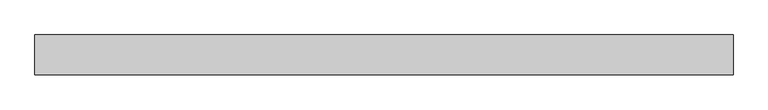
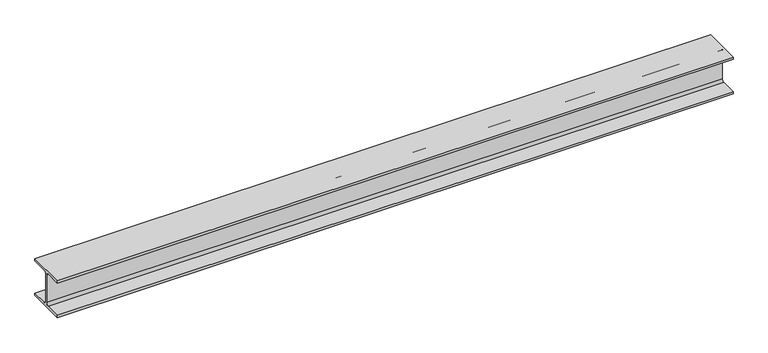
"""IFC4 building model written with IfcOpenShell, lengths in millimetres: beam geometry, 0912_Steel Framing_H-KSD3502 : H_SB_ASB_H-200x200x8x12."""

from ifc_helpers import new_model, si_unit, point, frame, frame_2d, origin, place, context, project, spatial, polyline, circle_curve, trimmed, segment, composite_curve, outline, extrude, source, transform, mapped, element, save


def beam_79464321(model_context):
    return source(origin(), model_context, "Body", "SweptSolid", [
        extrude(outline(composite_curve([segment(polyline([(100.0, -88.0), (100.0, -100.0), (-100.0, -100.0), (-100.0, -88.0), (-17.0, -88.0)]), True, "CONTINUOUS"), segment(trimmed(circle_curve(frame_2d((-17.0, -75.0)), 13.0), [point((-17.0, -88.0))], [point((-4.0, -75.0))], True, "CARTESIAN"), True, "CONTINUOUS"), segment(polyline([(-4.0, -75.0), (-4.0, 75.0)]), True, "CONTINUOUS"), segment(trimmed(circle_curve(frame_2d((-17.0, 75.0)), 13.0), [point((-4.0, 75.0))], [point((-17.0, 88.0))], True, "CARTESIAN"), True, "CONTINUOUS"), segment(polyline([(-17.0, 88.0), (-100.0, 88.0), (-100.0, 100.0), (100.0, 100.0), (100.0, 88.0), (17.0, 88.0)]), True, "CONTINUOUS"), segment(trimmed(circle_curve(frame_2d((17.0, 75.0)), 13.0), [point((17.0, 88.0))], [point((4.0, 75.0))], True, "CARTESIAN"), True, "CONTINUOUS"), segment(polyline([(4.0, 75.0), (4.0, -75.0)]), True, "CONTINUOUS"), segment(trimmed(circle_curve(frame_2d((17.0, -75.0)), 13.0), [point((4.0, -75.0))], [point((17.0, -88.0))], True, "CARTESIAN"), True, "CONTINUOUS"), segment(polyline([(17.0, -88.0), (100.0, -88.0)]), True, "CONTINUOUS")], self_intersect=False)), frame((-1792.5090133, 0.0, 0.0), z_axis=(1.0, 0.0, 0.0), x_axis=(0.0, 1.0, 0.0)), (0.0, 0.0, 1.0), 3485.497556),
    ])


if __name__ == "__main__":
    model = new_model("IFC4")
    model_context = context("Model", 3, world=origin())
    ifc_project = project(units=[si_unit("LENGTHUNIT", "METRE", prefix="MILLI")], contexts=[model_context])
    site = spatial("IfcSite", under=ifc_project)
    building = spatial("IfcBuilding", under=site)
    placement = place(None, origin())
    beam_shape = beam_79464321(model_context)
    element("IfcBeam", 1, ObjectType="0912_Steel Framing_H-KSD3502 : H_SB_ASB_H-200x200x8x12", at=placement, inside=building, context=model_context, shape_type="MappedRepresentation", body=[
        mapped(beam_shape, transform((0.0, 0.0, 0.0), x_axis=(1.0, 0.0, 0.0), y_axis=(0.0, 1.0, 0.0), z_axis=(0.0, 0.0, 1.0))),
    ])
    save(model, "model.ifc")

# Revit data of these elements
# Type "0912_Steel Framing_H-KSD3502 : H_SB_ASB_H-200x200x8x12"
#   H_WM Code_1 = "S01AA002-00001 | Main Steel Structure Fabrication Work | Shelter/Building | Medium Steel - Standard (90KG/M>Weight≥30KG/M) | Material: (   )"
#   H_WM Code_2 = "S03AA028-00001 | Main Steel Structure Erection Work | Shelter/Building | Medium Steel (90KG/M>Weight≥30KG/M) | Material: (   )"
#   H_WM Code_3 = "S01AA010-00001 | Main Steel Structure Fabrication Work | Shelter/Building | Steel Painting/Coating | for Non-Fireproofed Steel Surface, Surface Preparation, Primer, Second & Final Coat | Material: (   )"
#   H_Q'ty Cal Type Tag = "SB-Q2"
#   Width = 20.0 cm
#   Web Thickness = 0.8 cm
#   Web Fillet = 1.3 cm
#   Warping Constant = 141000.0 cm⁶
#   W = 0
#   Torsional Moment of Inertia = 26.2485 cm⁴
#   Section Area = 63.53 cm²
#   Plastic Modulus weak axis = 244.0 cm³
#   Plastic Modulus strong axis = 525.0 cm³
#   Perimeter = 1.16 m²/m
#   Nominal Weight = 49.90 kgf/m
#   Moment of Inertia weak axis = 1600.00 cm⁴
#   Moment of Inertia strong axis = 4720.00 cm⁴
#   Height = 20.0 cm
#   Flange Thickness = 1.2 cm
#   Elastic Modulus weak axis = 160.0 cm³
#   Elastic Modulus strong axis = 472.0 cm³
#   Centroid Vertical = 10.0 cm
#   Centroid Horizontal = 10.0 cm
#   Ix = 47200000
#   Length [instance default] = 1.5240 m
#   Zx = 525000
#   b = 0.2000 m
#   h = 0.2000 m
#   r = 0.0130 m
#   s = 0.0080 m
#   t = 0.0120 m
#   A = 0.006353 m²
#   Structural Material [instance default] = Steel, 45-345
#   Assembly Code = ""
# Element 1 (IfcBeam, "0912_Steel Framing_H-KSD3502 : H_SB_ASB_H-200x200x8x12")
#   Structural Material = none
# Materials
#   "Steel, 45-345": class "Metal", colour RGB 189 187 185, transparency 0, Description = "Steel 345 MPa", Cost = 0
